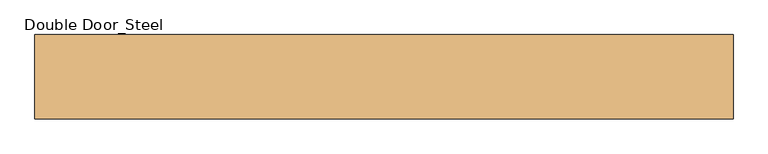
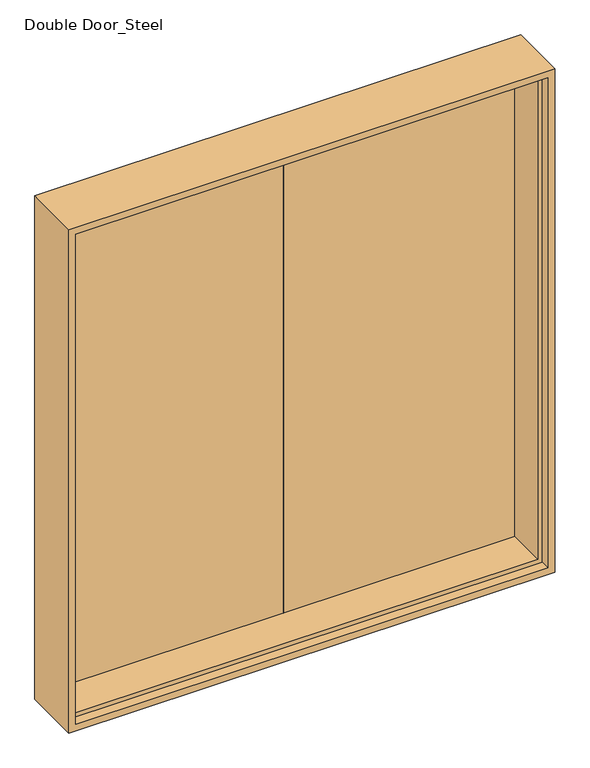
"""IFC4 building model written with IfcOpenShell, lengths in millimetres: door geometry, Double Door_Steel : H_DR_AR B12_Door_Double_W2100xH2280_No FR_SD-3."""

from ifc_helpers import new_model, si_unit, frame, origin, place, context, project, spatial, polyline, outline, extrude, faceted_brep, source, transform, mapped, element, save


def double_door_steel_deb95cd2(model_context):
    return source(origin(), model_context, "Body", "SolidModel", [
        faceted_brep([(1035.0, -125.0, 2265.0), (1035.0, 125.0, 2265.0), (-1035.0, 125.0, 2265.0), (-1035.0, -125.0, 2265.0), (985.0, 85.0, 2215.0), (985.0, -85.0, 2215.0), (-985.0, -85.0, 2215.0), (-985.0, 85.0, 2215.0), (1005.0, 125.0, 2235.0), (1005.0, 85.0, 2235.0), (-1005.0, 85.0, 2235.0), (-1005.0, 125.0, 2235.0), (-1035.0, 125.0, 0.0), (-1035.0, -125.0, 0.0), (-985.0, -85.0, 50.0), (-985.0, 85.0, 50.0), (-1005.0, 85.0, 30.0), (-1005.0, 125.0, 30.0), (1035.0, 125.0, 0.0), (1005.0, 125.0, 30.0), (1035.0, -125.0, 0.0), (1005.0, -125.0, 30.0), (-1005.0, -125.0, 30.0), (-1005.0, -125.0, 2235.0), (1005.0, -125.0, 2235.0), (985.0, -85.0, 50.0), (985.0, 85.0, 50.0), (1005.0, 85.0, 30.0), (1005.0, -85.0, 2235.0), (-1005.0, -85.0, 2235.0), (-1005.0, -85.0, 30.0), (1005.0, -85.0, 30.0)], [[[0, 1, 2, 3]], [[4, 5, 6, 7]], [[8, 9, 10, 11]], [[3, 2, 12, 13]], [[7, 6, 14, 15]], [[11, 10, 16, 17]], [[18, 12, 2, 1], [8, 11, 17, 19]], [[13, 12, 18, 20]], [[0, 3, 13, 20], [21, 22, 23, 24]], [[15, 14, 25, 26]], [[27, 16, 10, 9], [4, 7, 15, 26]], [[17, 16, 27, 19]], [[20, 18, 1, 0]], [[26, 25, 5, 4]], [[19, 27, 9, 8]], [[28, 24, 23, 29]], [[29, 23, 22, 30]], [[30, 22, 21, 31]], [[31, 21, 24, 28]], [[29, 30, 31, 28], [5, 25, 14, 6]]]),
        extrude(outline(polyline([(1005.0, 85.0), (0.0, 85.0), (0.0, 125.0), (1005.0, 125.0), (1005.0, 85.0)])), frame((0.0, 0.0, 30.0), z_axis=(0.0, 0.0, 1.0), x_axis=(1.0, 0.0, 0.0)), (0.0, 0.0, 1.0), 2205.0),
        extrude(outline(polyline([(0.0, 85.0), (-1005.0, 85.0), (-1005.0, 125.0), (0.0, 125.0), (0.0, 85.0)])), frame((0.0, 0.0, 30.0), z_axis=(0.0, 0.0, 1.0), x_axis=(1.0, 0.0, 0.0)), (0.0, 0.0, 1.0), 2205.0),
    ])


if __name__ == "__main__":
    model = new_model("IFC4")
    model_context = context("Model", 3, world=origin())
    ifc_project = project(units=[si_unit("LENGTHUNIT", "METRE", prefix="MILLI")], contexts=[model_context])
    site = spatial("IfcSite", under=ifc_project)
    building = spatial("IfcBuilding", under=site)
    placement = place(None, origin())
    double_door_steel_shape = double_door_steel_deb95cd2(model_context)
    element("IfcDoor", 1, ObjectType="Double Door_Steel : H_DR_AR B12_Door_Double_W2100xH2280_No FR_SD-3", at=placement, inside=building, context=model_context, shape_type="MappedRepresentation", body=[
        mapped(double_door_steel_shape, transform((0.0, 0.0, 0.0), x_axis=(1.0, 0.0, 0.0), y_axis=(0.0, 1.0, 0.0), z_axis=(0.0, 0.0, 1.0))),
    ])
    save(model, "model.ifc")

# Revit data of these elements
# Type "Double Door_Steel : H_DR_AR B12_Door_Double_W2100xH2280_No FR_SD-3"
#   Type Mark = "439"
#   프레임 = ""
#   철물 = ""
#   유리/마감 = ""
#   위치/개소 = ""
#   부호 = ""
#   문번호 = ""
#   문기호 = "SD-3"
#   Analytic Construction = "<None>"
#   Door Width = 1005 mm
#   Height = 2280 mm
#   Width = 2100 mm
#   Define Thermal Properties by = 1
#   문 틀 = none
#   문 = none
#   Function = (empty or 0)
#   Assembly Code = ""
#   Wall Closure = (empty or 0)
